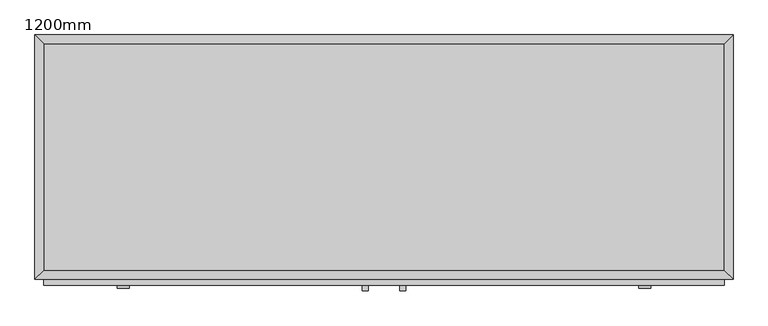
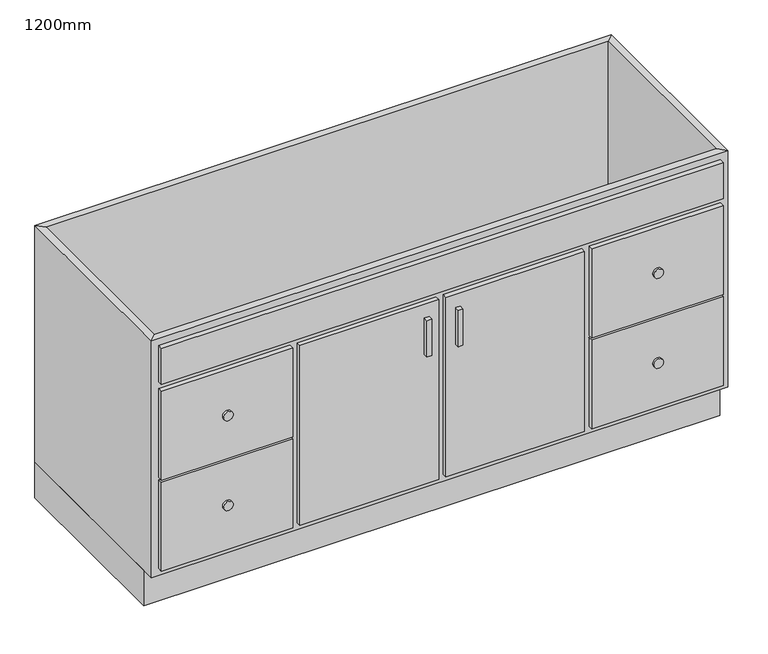
"""IFC4 building model written with IfcOpenShell, lengths in millimetres: furniture geometry, M_Vanity Cabinet-Double Door & 4 Drawer : 1200mm."""

from ifc_helpers import new_model, si_unit, point, frame, frame_2d, origin, origin_with_axes, place, context, project, spatial, polyline, circle_curve, trimmed, segment, composite_curve, outline, extrude, faceted_brep, source, transform, mapped, element, save


def furniture_1200mm_7f9456d8(model_context):
    return source(origin(), model_context, "Body", "SolidModel", [
        extrude(outline(polyline([(55.91996, -558.8), (43.21996, -558.8), (43.21996, -546.1), (55.91996, -546.1), (55.91996, -558.8)])), frame((0.0, 0.0, 482.6), z_axis=(0.0, 0.0, 1.0), x_axis=(1.0, 0.0, 0.0)), (0.0, 0.0, 1.0), 101.6),
        extrude(outline(polyline([(138.46996, -558.8), (125.76996, -558.8), (125.76996, -546.1), (138.46996, -546.1), (138.46996, -558.8)])), frame((0.0, 0.0, 482.6), z_axis=(0.0, 0.0, 1.0), x_axis=(1.0, 0.0, 0.0)), (0.0, 0.0, 1.0), 101.6),
        extrude(outline(polyline([(833.79496, -546.1), (-652.10504, -546.1), (-652.10504, -533.4), (833.79496, -533.4), (833.79496, -546.1)])), frame((0.0, 0.0, 641.35), z_axis=(0.0, 0.0, 1.0), x_axis=(1.0, 0.0, 0.0)), (0.0, 0.0, 1.0), 101.6),
        extrude(outline(polyline([(833.79496, -546.1), (486.13246, -546.1), (486.13246, -533.4), (833.79496, -533.4), (833.79496, -546.1)])), frame((0.0, 0.0, 373.85), z_axis=(0.0, 0.0, 1.0), x_axis=(1.0, 0.0, 0.0)), (0.0, 0.0, 1.0), 248.45),
        extrude(outline(polyline([(833.79496, -546.1), (486.13246, -546.1), (486.13246, -533.4), (833.79496, -533.4), (833.79496, -546.1)])), frame((0.0, 0.0, 119.05), z_axis=(0.0, 0.0, 1.0), x_axis=(1.0, 0.0, 0.0)), (0.0, 0.0, 1.0), 248.45),
        extrude(outline(polyline([(-304.44254, -546.1), (-652.10504, -546.1), (-652.10504, -533.4), (-304.44254, -533.4), (-304.44254, -546.1)])), frame((0.0, 0.0, 373.85), z_axis=(0.0, 0.0, 1.0), x_axis=(1.0, 0.0, 0.0)), (0.0, 0.0, 1.0), 248.45),
        extrude(outline(polyline([(-304.44254, -546.1), (-652.10504, -546.1), (-652.10504, -533.4), (-304.44254, -533.4), (-304.44254, -546.1)])), frame((0.0, 0.0, 119.05), z_axis=(0.0, 0.0, 1.0), x_axis=(1.0, 0.0, 0.0)), (0.0, 0.0, 1.0), 248.45),
        extrude(outline(polyline([(81.31996, -546.1), (-285.39254, -546.1), (-285.39254, -533.4), (81.31996, -533.4), (81.31996, -546.1)])), frame((0.0, 0.0, 119.05), z_axis=(0.0, 0.0, 1.0), x_axis=(1.0, 0.0, 0.0)), (0.0, 0.0, 1.0), 503.25),
        extrude(outline(polyline([(467.08246, -546.1), (100.36996, -546.1), (100.36996, -533.4), (467.08246, -533.4), (467.08246, -546.1)])), frame((0.0, 0.0, 119.05), z_axis=(0.0, 0.0, 1.0), x_axis=(1.0, 0.0, 0.0)), (0.0, 0.0, 1.0), 503.25),
        extrude(outline(composite_curve([segment(trimmed(circle_curve(frame_2d((496.4875, -478.27379)), 12.7), [point((496.4875, -490.97379))], [point((496.4875, -465.57379))], False, "CARTESIAN"), True, "CONTINUOUS"), segment(trimmed(circle_curve(frame_2d((496.4875, -478.27379)), 12.7), [point((496.4875, -465.57379))], [point((496.4875, -490.97379))], False, "CARTESIAN"), True, "CONTINUOUS")], self_intersect=False)), frame((0.0, -552.45, 0.0), z_axis=(0.0, 1.0, 0.0), x_axis=(0.0, 0.0, 1.0)), (0.0, 0.0, 1.0), 6.35),
        extrude(outline(composite_curve([segment(trimmed(circle_curve(frame_2d((244.8625, -478.27379)), 12.7), [point((244.8625, -490.97379))], [point((244.8625, -465.57379))], False, "CARTESIAN"), True, "CONTINUOUS"), segment(trimmed(circle_curve(frame_2d((244.8625, -478.27379)), 12.7), [point((244.8625, -465.57379))], [point((244.8625, -490.97379))], False, "CARTESIAN"), True, "CONTINUOUS")], self_intersect=False)), frame((0.0, -552.45, 0.0), z_axis=(0.0, 1.0, 0.0), x_axis=(0.0, 0.0, 1.0)), (0.0, 0.0, 1.0), 6.35),
        extrude(outline(composite_curve([segment(trimmed(circle_curve(frame_2d((244.8625, 659.96371)), 12.7), [point((244.8625, 647.26371))], [point((244.8625, 672.66371))], False, "CARTESIAN"), True, "CONTINUOUS"), segment(trimmed(circle_curve(frame_2d((244.8625, 659.96371)), 12.7), [point((244.8625, 672.66371))], [point((244.8625, 647.26371))], False, "CARTESIAN"), True, "CONTINUOUS")], self_intersect=False)), frame((0.0, -552.45, 0.0), z_axis=(0.0, 1.0, 0.0), x_axis=(0.0, 0.0, 1.0)), (0.0, 0.0, 1.0), 6.35),
        extrude(outline(composite_curve([segment(trimmed(circle_curve(frame_2d((496.4875, 659.96371)), 12.7), [point((496.4875, 647.26371))], [point((496.4875, 672.66371))], False, "CARTESIAN"), True, "CONTINUOUS"), segment(trimmed(circle_curve(frame_2d((496.4875, 659.96371)), 12.7), [point((496.4875, 672.66371))], [point((496.4875, 647.26371))], False, "CARTESIAN"), True, "CONTINUOUS")], self_intersect=False)), frame((0.0, -552.45, 0.0), z_axis=(0.0, 1.0, 0.0), x_axis=(0.0, 0.0, 1.0)), (0.0, 0.0, 1.0), 6.35),
        extrude(outline(polyline([(833.79496, -19.05), (833.79496, -514.35), (-652.10504, -514.35), (-652.10504, -19.05), (833.79496, -19.05)])), frame((0.0, 0.0, 100.0), z_axis=(0.0, 0.0, 1.0), x_axis=(1.0, 0.0, 0.0)), (0.0, 0.0, 1.0), 19.05),
        faceted_brep([(833.79496, -514.35, 762.0), (833.79496, -514.35, 100.0), (-652.10504, -514.35, 100.0), (-652.10504, -514.35, 762.0), (852.84496, -533.4, 762.0), (-671.15504, -533.4, 762.0), (852.84496, -533.4, 100.0), (-671.15504, -533.4, 100.0), (-652.10504, -19.05, 100.0), (-652.10504, -19.05, 762.0), (-671.15504, 0.0, 762.0), (-671.15504, 0.0, 100.0), (833.79496, -19.05, 100.0), (833.79496, -19.05, 762.0), (852.84496, 0.0, 762.0), (852.84496, 0.0, 100.0)], [[[0, 1, 2, 3]], [[4, 0, 3, 5]], [[6, 4, 5, 7]], [[1, 6, 7, 2]], [[3, 2, 8, 9]], [[5, 3, 9, 10]], [[7, 5, 10, 11]], [[2, 7, 11, 8]], [[9, 8, 12, 13]], [[10, 9, 13, 14]], [[11, 10, 14, 15]], [[8, 11, 15, 12]], [[13, 12, 1, 0]], [[14, 13, 0, 4]], [[15, 14, 4, 6]], [[12, 15, 6, 1]]]),
        extrude(outline(polyline([(852.84496, 0.0), (852.84496, -498.4), (-671.15504, -498.4), (-671.15504, 0.0), (852.84496, 0.0)])), origin_with_axes(), (0.0, 0.0, 1.0), 100.0),
    ])


if __name__ == "__main__":
    model = new_model("IFC4")
    model_context = context("Model", 3, world=origin())
    ifc_project = project(units=[si_unit("LENGTHUNIT", "METRE", prefix="MILLI")], contexts=[model_context])
    site = spatial("IfcSite", under=ifc_project)
    building = spatial("IfcBuilding", under=site)
    placement = place(None, origin())
    furniture_1200mm_shape = furniture_1200mm_7f9456d8(model_context)
    element("IfcFurniture", 1, ObjectType="M_Vanity Cabinet-Double Door & 4 Drawer : 1200mm", at=placement, inside=building, context=model_context, shape_type="MappedRepresentation", body=[
        mapped(furniture_1200mm_shape, transform((0.0, 0.0, 0.0), x_axis=(1.0, 0.0, 0.0), y_axis=(0.0, 1.0, 0.0), z_axis=(0.0, 0.0, 1.0))),
    ])
    save(model, "model.ifc")

# Revit data of these elements
# Type "M_Vanity Cabinet-Double Door & 4 Drawer : 1200mm"
#   Depth = 1' - 9"
#   Height = 2' - 6"
#   Plinth Depth = 0' - 1.37795"
#   Plinth Height = 0' - 3.93701"
#   Width = 5' - 0"
#   Cabinet Material = none
#   Door/Drawer Material = none
#   Handle Material = Cabinets - Handles
#   Default Elevation = 0
# Element 1 (IfcFurniture, "M_Vanity Cabinet-Double Door & 4 Drawer : 1200mm")
#   Materials on its faces: "Cabinets", "Cabinets - Handles"
# Materials
#   "Cabinets - Handles": class "Metal", colour RGB 57 57 57, transparency 0
#   "Cabinets": class "Miscellaneous", colour RGB 249 249 249, transparency 0
